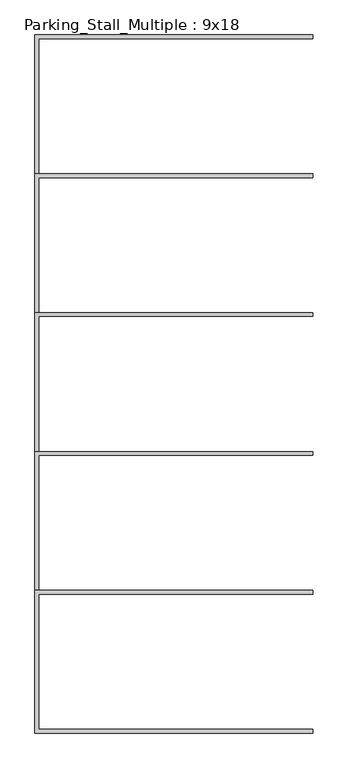
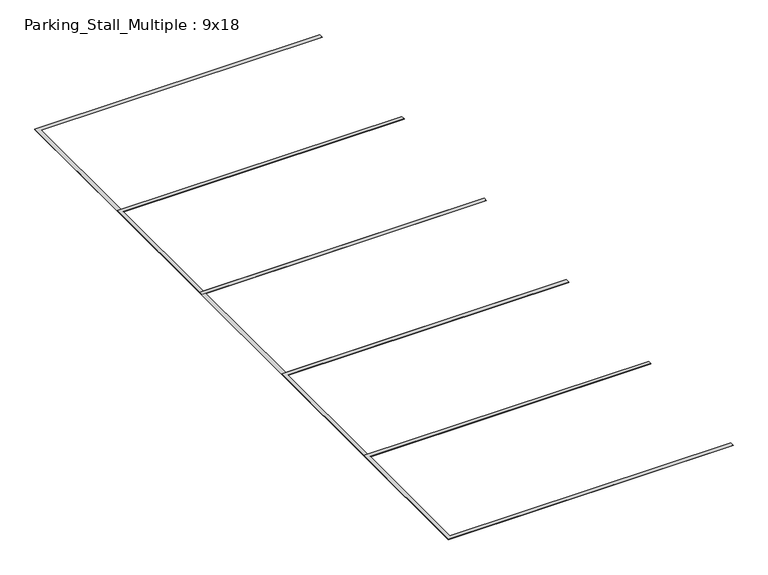
"""IFC4 building model written with IfcOpenShell, lengths in millimetres: proxy geometry, Parking_Stall_Multiple : 9x18."""

from ifc_helpers import new_model, si_unit, origin, origin_with_axes, place, context, project, spatial, polyline, outline, extrude, source, transform, mapped, element, save


def parking_stall_multiple_9x18_1f400319(model_context):
    return source(origin(), model_context, "Body", "SweptSolid", [
        extrude(outline(polyline([(5486.4, -10972.8), (5486.4, -11049.0), (76.2, -11049.0), (76.2, -13716.0), (5486.4, -13716.0), (5486.4, -13792.2), (0.0, -13792.2), (0.0, -10972.8), (5486.4, -10972.8)])), origin_with_axes(), (0.0, 0.0, 1.0), 6.35),
        extrude(outline(polyline([(5486.4, -8229.6), (5486.4, -8305.8), (76.2, -8305.8), (76.2, -10972.8), (5486.4, -10972.8), (5486.4, -11049.0), (0.0, -11049.0), (0.0, -8229.6), (5486.4, -8229.6)])), origin_with_axes(), (0.0, 0.0, 1.0), 6.35),
        extrude(outline(polyline([(5486.4, -5486.4), (5486.4, -5562.6), (76.2, -5562.6), (76.2, -8229.6), (5486.4, -8229.6), (5486.4, -8305.8), (0.0, -8305.8), (0.0, -5486.4), (5486.4, -5486.4)])), origin_with_axes(), (0.0, 0.0, 1.0), 6.35),
        extrude(outline(polyline([(5486.4, -2743.2), (5486.4, -2819.4), (76.2, -2819.4), (76.2, -5486.4), (5486.4, -5486.4), (5486.4, -5562.6), (0.0, -5562.6), (0.0, -2743.2), (5486.4, -2743.2)])), origin_with_axes(), (0.0, 0.0, 1.0), 6.35),
        extrude(outline(polyline([(5486.4, 0.0), (5486.4, -76.2), (76.2, -76.2), (76.2, -2743.2), (5486.4, -2743.2), (5486.4, -2819.4), (0.0, -2819.4), (0.0, 0.0), (5486.4, 0.0)])), origin_with_axes(), (0.0, 0.0, 1.0), 6.35),
    ])


if __name__ == "__main__":
    model = new_model("IFC4")
    model_context = context("Model", 3, world=origin())
    ifc_project = project(units=[si_unit("LENGTHUNIT", "METRE", prefix="MILLI")], contexts=[model_context])
    site = spatial("IfcSite", under=ifc_project)
    building = spatial("IfcBuilding", under=site)
    placement = place(None, origin())
    parking_stall_multiple_9x18_shape = parking_stall_multiple_9x18_1f400319(model_context)
    element("IfcBuildingElementProxy", 1, Name="Parking_Stall_Multiple : 9x18", ObjectType="Parking_Stall_Multiple : 9x18", at=placement, inside=building, context=model_context, shape_type="MappedRepresentation", body=[
        mapped(parking_stall_multiple_9x18_shape, transform((0.0, 0.0, 0.0), x_axis=(1.0, 0.0, 0.0), y_axis=(0.0, 1.0, 0.0), z_axis=(0.0, 0.0, 1.0))),
    ])
    save(model, "model.ifc")

# Revit data of these elements
# Type "Parking_Stall_Multiple : 9x18"
#   Parking_Width_M = 9' - 0"
#   Parking_Run_Length [instance default] = 65' - 0"
#   Parking_Line_Width = 0' - 3"
#   Parking_Length_M = 18' - 0"
#   Single_Parking_Visibility [instance default] = no
#   Parking_ADA_Symbol = no
#   ParkingUnitsArray [instance default] = 7
#   ParkingUnits [instance default] = 7
#   Multiple_Parking_Visibility [instance default] = yes
#   Parking_Line_Material = none
# Element 1 (IfcBuildingElementProxy, "Parking_Stall_Multiple : 9x18")
#   Parking_Run_Length = 45' - 4.43699"
#   ParkingUnitsArray = 5
#   ParkingUnits = 5
